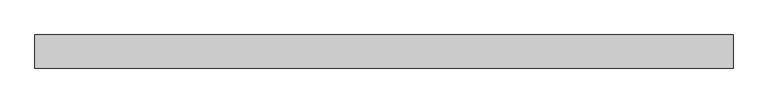
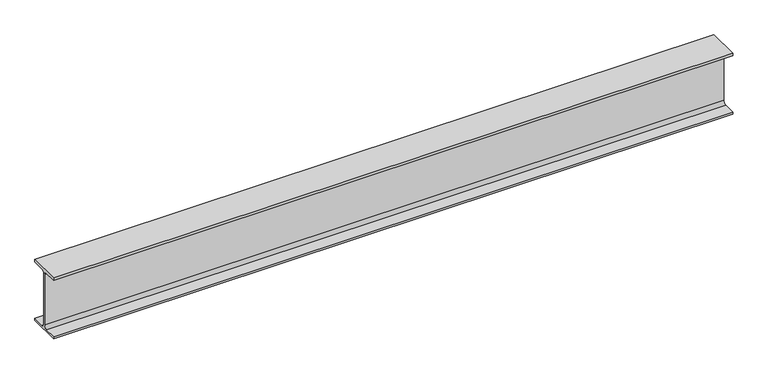
"""IFC4 building model written with IfcOpenShell, lengths in millimetres: beam geometry, 0912_Steel Framing_H-KSD3502 : H_SB_ASB_H-250x125x6x9."""

from ifc_helpers import new_model, si_unit, point, frame, frame_2d, origin, place, context, project, spatial, polyline, circle_curve, trimmed, segment, composite_curve, outline, extrude, source, transform, mapped, element, save


def beam_ec440c2a(model_context):
    return source(origin(), model_context, "Body", "SweptSolid", [
        extrude(outline(composite_curve([segment(polyline([(62.5, -116.0), (62.5, -125.0), (-62.5, -125.0), (-62.5, -116.0), (-15.0, -116.0)]), True, "CONTINUOUS"), segment(trimmed(circle_curve(frame_2d((-15.0, -104.0)), 12.0), [point((-15.0, -116.0))], [point((-3.0, -104.0))], True, "CARTESIAN"), True, "CONTINUOUS"), segment(polyline([(-3.0, -104.0), (-3.0, 104.0)]), True, "CONTINUOUS"), segment(trimmed(circle_curve(frame_2d((-15.0, 104.0)), 12.0), [point((-3.0, 104.0))], [point((-15.0, 116.0))], True, "CARTESIAN"), True, "CONTINUOUS"), segment(polyline([(-15.0, 116.0), (-62.5, 116.0), (-62.5, 125.0), (62.5, 125.0), (62.5, 116.0), (15.0, 116.0)]), True, "CONTINUOUS"), segment(trimmed(circle_curve(frame_2d((15.0, 104.0)), 12.0), [point((15.0, 116.0))], [point((3.0, 104.0))], True, "CARTESIAN"), True, "CONTINUOUS"), segment(polyline([(3.0, 104.0), (3.0, -104.0)]), True, "CONTINUOUS"), segment(trimmed(circle_curve(frame_2d((15.0, -104.0)), 12.0), [point((3.0, -104.0))], [point((15.0, -116.0))], True, "CARTESIAN"), True, "CONTINUOUS"), segment(polyline([(15.0, -116.0), (62.5, -116.0)]), True, "CONTINUOUS")], self_intersect=False)), frame((-1387.3, 0.0, 0.0), z_axis=(1.0, 0.0, 0.0), x_axis=(0.0, 1.0, 0.0)), (0.0, 0.0, 1.0), 2636.6),
    ])


if __name__ == "__main__":
    model = new_model("IFC4")
    model_context = context("Model", 3, world=origin())
    ifc_project = project(units=[si_unit("LENGTHUNIT", "METRE", prefix="MILLI")], contexts=[model_context])
    site = spatial("IfcSite", under=ifc_project)
    building = spatial("IfcBuilding", under=site)
    placement = place(None, origin())
    beam_shape = beam_ec440c2a(model_context)
    element("IfcBeam", 1, ObjectType="0912_Steel Framing_H-KSD3502 : H_SB_ASB_H-250x125x6x9", at=placement, inside=building, context=model_context, shape_type="MappedRepresentation", body=[
        mapped(beam_shape, transform((0.0, 0.0, 0.0), x_axis=(1.0, 0.0, 0.0), y_axis=(0.0, 1.0, 0.0), z_axis=(0.0, 0.0, 1.0))),
    ])
    save(model, "model.ifc")

# Revit data of these elements
# Type "0912_Steel Framing_H-KSD3502 : H_SB_ASB_H-250x125x6x9"
#   H_WM Code_1 = "S01AA003-00001 | Main Steel Structure Fabrication Work | Shelter/Building | Light Steel - Standard (30KG/M>Weight) | Material: (   )"
#   H_WM Code_2 = "S03AA029-00001 | Main Steel Structure Erection Work | Shelter/Building | Light Steel (30KG/M>Weight) | Material: (   )"
#   H_WM Code_3 = "S01AA010-00001 | Main Steel Structure Fabrication Work | Shelter/Building | Steel Painting/Coating | for Non-Fireproofed Steel Surface, Surface Preparation, Primer, Second & Final Coat | Material: (   )"
#   H_Q'ty Cal Type Tag = "SB-Q2"
#   Width = 12.5 cm
#   Web Thickness = 0.6 cm
#   Web Fillet = 1.2 cm
#   Warping Constant = 42539.8 cm⁶
#   W = 0
#   Torsional Moment of Inertia = 7.8102 cm⁴
#   Section Area = 37.66 cm²
#   Plastic Modulus weak axis = 73.1 cm³
#   Plastic Modulus strong axis = 366.0 cm³
#   Perimeter = 0.97 m²/m
#   Nominal Weight = 29.60 kgf/m
#   Moment of Inertia weak axis = 294.00 cm⁴
#   Moment of Inertia strong axis = 4050.00 cm⁴
#   Height = 25.0 cm
#   Flange Thickness = 0.9 cm
#   Elastic Modulus weak axis = 47.0 cm³
#   Elastic Modulus strong axis = 324.0 cm³
#   Centroid Vertical = 12.5 cm
#   Centroid Horizontal = 6.25 cm
#   Ix = 40500000
#   Length [instance default] = 1.5240 m
#   Zx = 366000
#   b = 0.1250 m
#   h = 0.2500 m
#   r = 0.0120 m
#   s = 0.0060 m
#   t = 0.0090 m
#   A = 0.003766 m²
#   Structural Material [instance default] = Steel, 45-345
#   Assembly Code = ""
# Element 1 (IfcBeam, "0912_Steel Framing_H-KSD3502 : H_SB_ASB_H-250x125x6x9")
#   Structural Material = none
# Materials
#   "Steel, 45-345": class "Metal", colour RGB 189 187 185, transparency 0, Description = "Steel 345 MPa", Cost = 0
